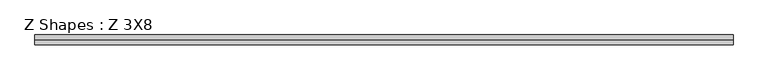
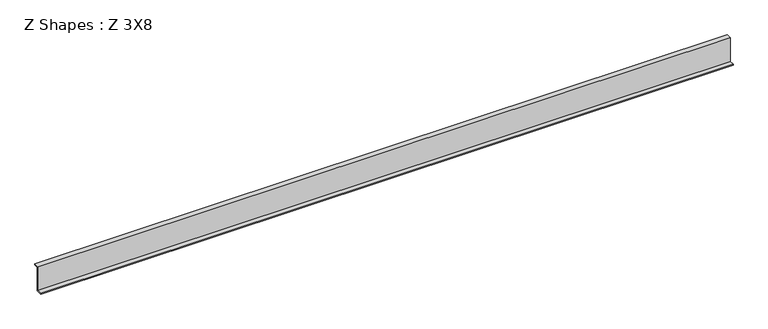
"""IFC4 building model written with IfcOpenShell, lengths in millimetres: beam geometry, Z Shapes : Z 3X8."""

import ifcopenshell
import ifcopenshell.guid

model = None  # the IFC model being written
_history = None  # IfcOwnerHistory: only IFC2X3 demands one
_inside = {}  # id of a spatial element -> (the spatial element, [elements in it])
_under = {}  # id of a project, library or spatial element -> (it, [spatial elements below it])
_declared = {}  # id of a project -> (the project, [libraries it declares])
_typed = {}  # id of a type object -> (the type object, [elements of that type])
_made_of = {}  # id of a material, layer set ... -> (it, [elements and type objects made of it])


def new_model(schema):
    """Start an empty IFC model of exactly this schema.

    Asked for "IFC4X3", IfcOpenShell would pick the latest addendum, in which some entities
    have other attributes; the version numbers below select the first issue.
    IFC2X3 requires an IfcOwnerHistory on every rooted entity: one is made here for all.
    """
    global model, _history
    if schema == "IFC4X3":
        model = ifcopenshell.file(schema_version=(4, 3, 0, 0))
    else:
        model = ifcopenshell.file(schema=schema)
    _inside.clear()
    _under.clear()
    _declared.clear()
    _typed.clear()
    _made_of.clear()
    _history = None
    if model.schema == "IFC2X3":
        org = make("IfcOrganization", Name="unknown")
        user = make(
            "IfcPersonAndOrganization",
            ThePerson=make("IfcPerson", FamilyName="unknown"),
            TheOrganization=org,
        )
        app = make(
            "IfcApplication",
            ApplicationDeveloper=org,
            Version="unknown",
            ApplicationFullName="unknown",
            ApplicationIdentifier="unknown",
        )
        _history = make(
            "IfcOwnerHistory",
            OwningUser=user,
            OwningApplication=app,
            ChangeAction="ADDED",
            CreationDate=0,
        )
    return model


def make(cls, **values):
    """One entity of the class cls with the attributes given. An attribute that is None is left unset."""
    return model.create_entity(
        cls, **{name: value for name, value in values.items() if value is not None}
    )


def rooted(cls, **values):
    """An entity with a GlobalId (a new one), such as an element, a storey or a relation."""
    return make(cls, GlobalId=ifcopenshell.guid.new(), OwnerHistory=_history, **values)


def si_unit(unit_type, name, prefix=None):
    """IfcSIUnit, for example si_unit("LENGTHUNIT", "METRE", prefix="MILLI")."""
    return make("IfcSIUnit", UnitType=unit_type, Prefix=prefix, Name=name)


def assignment(units):
    """IfcUnitAssignment: the units of a project."""
    return None if units is None else make("IfcUnitAssignment", Units=units)


def point(xyz):
    """IfcCartesianPoint."""
    return None if xyz is None else make("IfcCartesianPoint", Coordinates=xyz)


def direction(xyz):
    """IfcDirection."""
    return None if xyz is None else make("IfcDirection", DirectionRatios=xyz)


def frame(location, z_axis=None, x_axis=None):
    """IfcAxis2Placement3D, a coordinate frame: its origin and axes. An axis left out is left unset."""
    return make(
        "IfcAxis2Placement3D",
        Location=point(location),
        Axis=direction(z_axis),
        RefDirection=direction(x_axis),
    )


def origin():
    """The frame at (0, 0, 0) with its axes left unset."""
    return frame((0.0, 0.0, 0.0))


def place(relative_to, where):
    """IfcLocalPlacement: puts the frame where relative to a parent placement (None: the world)."""
    return make(
        "IfcLocalPlacement", PlacementRelTo=relative_to, RelativePlacement=where
    )


def context(
    kind, dimensions, precision=None, world=None, true_north=None, identifier=None
):
    """IfcGeometricRepresentationContext, for example the 3D "Model" context."""
    return make(
        "IfcGeometricRepresentationContext",
        ContextIdentifier=identifier,
        ContextType=kind,
        CoordinateSpaceDimension=dimensions,
        Precision=precision,
        WorldCoordinateSystem=world,
        TrueNorth=true_north,
    )


def project(units=None, contexts=None):
    """IfcProject with its units and contexts."""
    return rooted(
        "IfcProject",
        Name="project",
        RepresentationContexts=contexts,
        UnitsInContext=assignment(units),
    )


def spatial(cls, under=None, at=None, **own):
    """A site, building, storey or space (cls), placed at a placement, below another one or the project."""
    s = rooted(cls, ObjectPlacement=at, **own)
    if under is not None:
        _under.setdefault(under.id(), (under, []))[1].append(s)
    return s


def polyline(points):
    """IfcPolyline through the points."""
    return make("IfcPolyline", Points=[point(p) for p in points])


def outline(outer, holes=None, kind="AREA"):
    """IfcArbitraryClosedProfileDef: a profile drawn as a closed curve; with holes, ...WithVoids."""
    if holes is None:
        return make("IfcArbitraryClosedProfileDef", ProfileType=kind, OuterCurve=outer)
    return make(
        "IfcArbitraryProfileDefWithVoids",
        ProfileType=kind,
        OuterCurve=outer,
        InnerCurves=holes,
    )


def extrude(swept, where, along, depth):
    """IfcExtrudedAreaSolid: the profile swept, set in the frame where, extruded along a direction by depth."""
    return make(
        "IfcExtrudedAreaSolid",
        SweptArea=swept,
        Position=where,
        ExtrudedDirection=direction(along),
        Depth=depth,
    )


def shape(context_of_items, identifier, shape_type, items):
    """IfcShapeRepresentation: the items that make up one representation, for example the "Body"."""
    return make(
        "IfcShapeRepresentation",
        ContextOfItems=context_of_items,
        RepresentationIdentifier=identifier,
        RepresentationType=shape_type,
        Items=items,
    )


def source(mapping_origin, context_of_items, identifier, shape_type, items):
    """IfcRepresentationMap: a shape defined once, which mapped items show again and again."""
    return make(
        "IfcRepresentationMap",
        MappingOrigin=mapping_origin,
        MappedRepresentation=shape(context_of_items, identifier, shape_type, items),
    )


def transform(
    local_origin,
    x_axis=None,
    y_axis=None,
    z_axis=None,
    scale=None,
    scale2=None,
    scale3=None,
    uniform=True,
):
    """IfcCartesianTransformationOperator3D, or its non-uniform kind. x_axis, y_axis, z_axis: its Axis1, 2, 3."""
    if uniform:
        return make(
            "IfcCartesianTransformationOperator3D",
            Axis1=direction(x_axis),
            Axis2=direction(y_axis),
            LocalOrigin=point(local_origin),
            Scale=scale,
            Axis3=direction(z_axis),
        )
    return make(
        "IfcCartesianTransformationOperator3DnonUniform",
        Axis1=direction(x_axis),
        Axis2=direction(y_axis),
        LocalOrigin=point(local_origin),
        Scale=scale,
        Axis3=direction(z_axis),
        Scale2=scale2,
        Scale3=scale3,
    )


def mapped(mapping_source, mapping_target):
    """IfcMappedItem: shows the shape of a source again, moved by a transform."""
    return make(
        "IfcMappedItem", MappingSource=mapping_source, MappingTarget=mapping_target
    )


def made_of(thing, what):
    """Note that an element or type object is made of a material, layer set ...; save() writes the relation."""
    if what is not None:
        _made_of.setdefault(what.id(), (what, []))[1].append(thing)
    return thing


def element(
    cls,
    number,
    at=None,
    inside=None,
    cuts=None,
    type_object=None,
    material=None,
    context=None,
    identifier="Body",
    shape_type=None,
    held_by="IfcProductDefinitionShape",
    body=None,
    shapes=None,
    **own,
):
    """One element of the class cls, such as IfcWall. Its Tag is "e" and its number.

    at: its placement. inside: the storey or other place that contains it. cuts: it is an
    opening in that element (IfcRelVoidsElement). A single representation is given by context,
    identifier, shape_type and body (its items); several are given by shapes. held_by: the class
    of the entity that holds the representations. save() writes the other relations.
    """
    e = rooted(cls, Tag="e%d" % number, ObjectPlacement=at, **own)
    if body is not None:
        shapes = [shape(context, identifier, shape_type, body)]
    if shapes is not None:
        e.Representation = make(held_by, Representations=shapes)
    if inside is not None:
        _inside.setdefault(inside.id(), (inside, []))[1].append(e)
    if cuts is not None:
        rooted(
            "IfcRelVoidsElement", RelatingBuildingElement=cuts, RelatedOpeningElement=e
        )
    if type_object is not None:
        _typed.setdefault(type_object.id(), (type_object, []))[1].append(e)
    return made_of(e, material)


def aggregate(whole, parts):
    """IfcRelAggregates: a whole, such as a stair, and the parts it consists of."""
    return rooted("IfcRelAggregates", RelatingObject=whole, RelatedObjects=parts)


def save(model, path):
    """Write the relations noted so far, then the file.

    IfcRelAggregates (storeys below a building ...), IfcRelContainedInSpatialStructure (elements
    in a storey), IfcRelDefinesByType, IfcRelAssociatesMaterial and IfcRelDeclares: one each for
    every whole, place, type object, material and project.
    """
    for whole, parts in _under.values():
        aggregate(whole, parts)
    for where, things in _inside.values():
        rooted(
            "IfcRelContainedInSpatialStructure",
            RelatedElements=things,
            RelatingStructure=where,
        )
    for kind, things in _typed.values():
        rooted("IfcRelDefinesByType", RelatedObjects=things, RelatingType=kind)
    for what, things in _made_of.values():
        rooted("IfcRelAssociatesMaterial", RelatedObjects=things, RelatingMaterial=what)
    for by, libraries in _declared.values():
        rooted("IfcRelDeclares", RelatingContext=by, RelatedDefinitions=libraries)
    model.write(path)


def z_shapes_z_3x8_3d6c6c97(model_context):
    return source(origin(), model_context, "Body", "SweptSolid", [
        extrude(outline(polyline([(57.2805719, 92.452825), (27.1991352, 92.452825), (27.1991352, -98.809175), (-18.9194281, -98.809175), (-18.9194281, -92.459175), (19.1805719, -92.459175), (19.1805719, 102.104825), (57.2805719, 102.104825), (57.2805719, 92.452825)])), frame((-2667.0, 0.0, 0.0), z_axis=(1.0, 0.0, 0.0), x_axis=(0.0, 1.0, 0.0)), (0.0, 0.0, 1.0), 5334.0),
    ])


if __name__ == "__main__":
    model = new_model("IFC4")
    model_context = context("Model", 3, world=origin())
    ifc_project = project(units=[si_unit("LENGTHUNIT", "METRE", prefix="MILLI")], contexts=[model_context])
    site = spatial("IfcSite", under=ifc_project)
    building = spatial("IfcBuilding", under=site)
    placement = place(None, origin())
    z_shapes_z_3x8_shape = z_shapes_z_3x8_3d6c6c97(model_context)
    element("IfcBeam", 1, ObjectType="Z Shapes : Z 3X8", at=placement, inside=building, context=model_context, shape_type="MappedRepresentation", body=[
        mapped(z_shapes_z_3x8_shape, transform((0.0, 0.0, 0.0), x_axis=(1.0, 0.0, 0.0), y_axis=(0.0, 1.0, 0.0), z_axis=(0.0, 0.0, 1.0))),
    ])
    save(model, "model.ifc")

# Revit data of these elements
# Type "Z Shapes : Z 3X8"
#   Section Name Key = "W12x26"
#   Assembly Code = "B10"
#   Width = 76.2 mm
#   Web Thickness = 5.842 mm
#   Web Fillet = 7.62 mm
#   Warping Constant = 163001.3 cm⁶
#   Torsional Moment of Inertia = 12.4869 cm⁴
#   Section Area = 7.65 in²
#   Plastic Modulus weak axis = 0.00472801 (stored number, unit not read)
#   Plastic Modulus strong axis = 0.0215278 (stored number, unit not read)
#   Perimeter = 15.0571 m²/m
#   Nominal Weight = 379.441 N/m
#   Moment of Inertia weak axis = 720.08 cm⁴
#   Moment of Inertia strong axis = 8491.12 cm⁴
#   Height = 184.912 mm
#   Flange Thickness = 9.652 mm
#   Elastic Modulus weak axis = 0.00309028 (stored number, unit not read)
#   Elastic Modulus strong axis = 0.0193287 (stored number, unit not read)
#   Centroid Vertical = 92.456 mm
#   Centroid Horizontal = 38.1 mm
#   Length [instance default] = 5' - 0"
#   Structural Material [instance default] = Steel ASTM A992
#   Principal Axes Angle = 0
# Element 1 (IfcBeam, "Z Shapes : Z 3X8")
#   Structural Material = accent 2
#   Materials on its faces: "accent 2"
# Materials
#   "Steel ASTM A992": class "Metal", colour RGB 189 187 185, transparency 0, Description = "Structural steel 50ksi", Cost = 0
#   "accent 2": class "Wood", colour RGB 80 80 80, transparency 0, Description = "Wood framing, thermal airspace", Cost = 0
